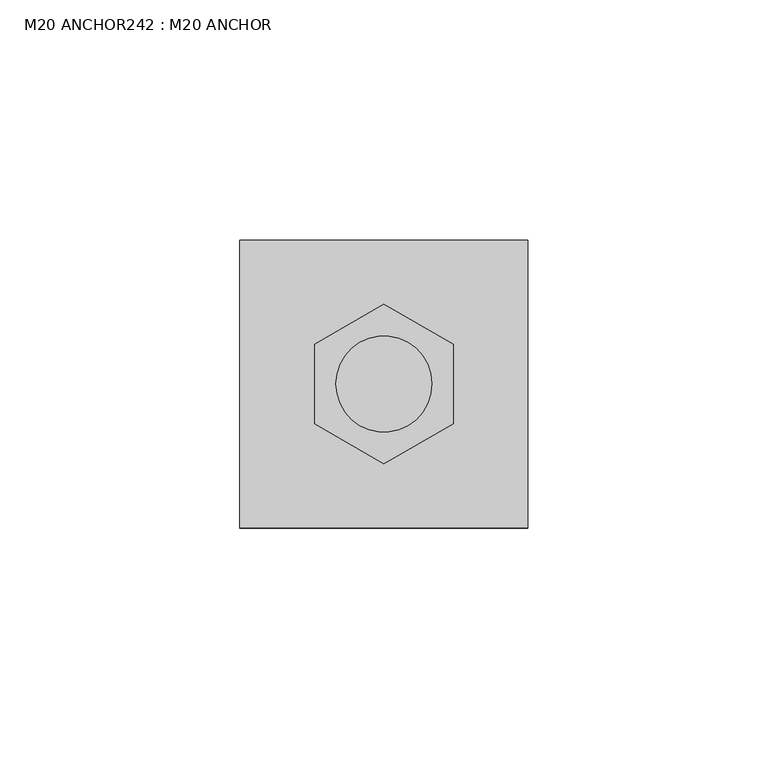
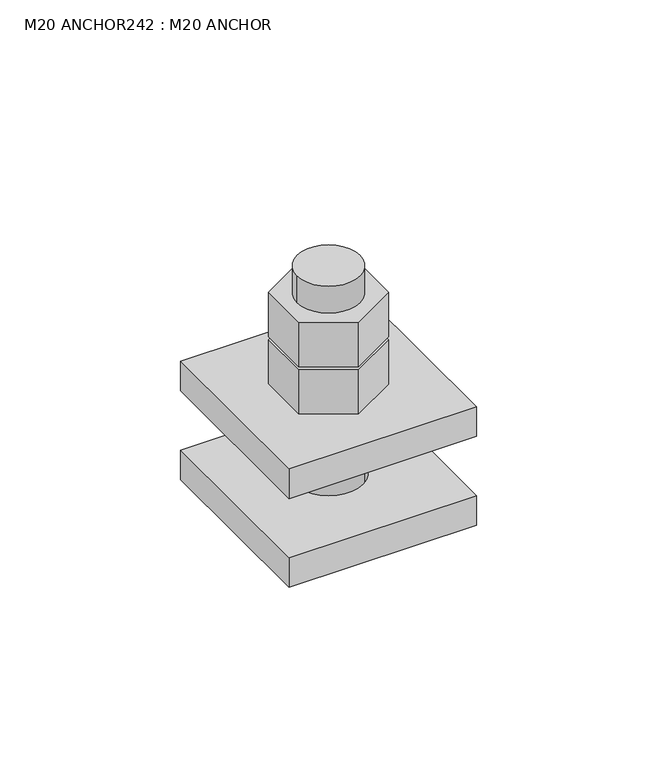
"""IFC4 building model written with IfcOpenShell, lengths in millimetres: fastener geometry, M20 ANCHOR242 : M20 ANCHOR."""

from ifc_helpers import new_model, si_unit, point, frame, frame_2d, origin, place, context, project, spatial, polyline, circle_curve, trimmed, segment, composite_curve, outline, extrude, source, transform, mapped, element, save


def m20_anchor242_m20_anchor_8256c240(model_context):
    return source(origin(), model_context, "Body", "SweptSolid", [
        extrude(outline(polyline([(9008.0855968, 22453.9464399), (9008.0855968, 22470.5835027), (9022.4937158, 22478.9020341), (9036.9018348, 22470.5835027), (9036.9018348, 22453.9464399), (9022.4937158, 22445.6279085), (9008.0855968, 22453.9464399)]), holes=[composite_curve([segment(trimmed(circle_curve(frame_2d((9022.4937158, 22462.2649713)), 10.0), [point((9032.4937158, 22462.2649713))], [point((9012.4937158, 22462.2649713))], True, "CARTESIAN"), True, "CONTINUOUS"), segment(trimmed(circle_curve(frame_2d((9022.4937158, 22462.2649713)), 10.0), [point((9012.4937158, 22462.2649713))], [point((9032.4937158, 22462.2649713))], True, "CARTESIAN"), True, "CONTINUOUS")], self_intersect=False)]), frame((0.0, 0.0, 246.0), z_axis=(0.0, 0.0, 1.0), x_axis=(1.0, 0.0, 0.0)), (0.0, 0.0, 1.0), 15.0),
        extrude(outline(polyline([(9008.0855968, 22453.9464399), (9008.0855968, 22470.5835027), (9022.4937158, 22478.9020341), (9036.9018348, 22470.5835027), (9036.9018348, 22453.9464399), (9022.4937158, 22445.6279085), (9008.0855968, 22453.9464399)]), holes=[composite_curve([segment(trimmed(circle_curve(frame_2d((9022.4937158, 22462.2649713)), 10.0), [point((9032.4937158, 22462.2649713))], [point((9012.4937158, 22462.2649713))], True, "CARTESIAN"), True, "CONTINUOUS"), segment(trimmed(circle_curve(frame_2d((9022.4937158, 22462.2649713)), 10.0), [point((9012.4937158, 22462.2649713))], [point((9032.4937158, 22462.2649713))], True, "CARTESIAN"), True, "CONTINUOUS")], self_intersect=False)]), frame((0.0, 0.0, 230.0), z_axis=(0.0, 0.0, 1.0), x_axis=(1.0, 0.0, 0.0)), (0.0, 0.0, 1.0), 15.0),
        extrude(outline(composite_curve([segment(trimmed(circle_curve(frame_2d((9022.4937158, 22462.2649713)), 10.0), [point((9032.4937158, 22462.2649713))], [point((9012.4937158, 22462.2649713))], False, "CARTESIAN"), True, "CONTINUOUS"), segment(trimmed(circle_curve(frame_2d((9022.4937158, 22462.2649713)), 10.0), [point((9012.4937158, 22462.2649713))], [point((9032.4937158, 22462.2649713))], False, "CARTESIAN"), True, "CONTINUOUS")], self_intersect=False)), frame((0.0, 0.0, 190.0), z_axis=(0.0, 0.0, 1.0), x_axis=(1.0, 0.0, 0.0)), (0.0, 0.0, 1.0), 80.0),
        extrude(outline(polyline([(8992.4937158, 22432.2649713), (8992.4937158, 22492.2649713), (9052.4937158, 22492.2649713), (9052.4937158, 22432.2649713), (8992.4937158, 22432.2649713)]), holes=[composite_curve([segment(trimmed(circle_curve(frame_2d((9022.4937158, 22462.2649713)), 11.0), [point((9033.4937158, 22462.2649713))], [point((9011.4937158, 22462.2649713))], True, "CARTESIAN"), True, "CONTINUOUS"), segment(trimmed(circle_curve(frame_2d((9022.4937158, 22462.2649713)), 11.0), [point((9011.4937158, 22462.2649713))], [point((9033.4937158, 22462.2649713))], True, "CARTESIAN"), True, "CONTINUOUS")], self_intersect=False)]), frame((0.0, 0.0, 190.0), z_axis=(0.0, 0.0, 1.0), x_axis=(1.0, 0.0, 0.0)), (0.0, 0.0, 1.0), 10.0),
        extrude(outline(polyline([(8992.4937158, 22432.2649713), (8992.4937158, 22492.2649713), (9052.4937158, 22492.2649713), (9052.4937158, 22432.2649713), (8992.4937158, 22432.2649713)]), holes=[composite_curve([segment(trimmed(circle_curve(frame_2d((9022.4937158, 22462.2649713)), 11.0), [point((9033.4937158, 22462.2649713))], [point((9011.4937158, 22462.2649713))], True, "CARTESIAN"), True, "CONTINUOUS"), segment(trimmed(circle_curve(frame_2d((9022.4937158, 22462.2649713)), 11.0), [point((9011.4937158, 22462.2649713))], [point((9033.4937158, 22462.2649713))], True, "CARTESIAN"), True, "CONTINUOUS")], self_intersect=False)]), frame((0.0, 0.0, 220.0), z_axis=(0.0, 0.0, 1.0), x_axis=(1.0, 0.0, 0.0)), (0.0, 0.0, 1.0), 10.0),
    ])


if __name__ == "__main__":
    model = new_model("IFC4")
    model_context = context("Model", 3, world=origin())
    ifc_project = project(units=[si_unit("LENGTHUNIT", "METRE", prefix="MILLI")], contexts=[model_context])
    site = spatial("IfcSite", under=ifc_project)
    building = spatial("IfcBuilding", under=site)
    placement = place(None, origin())
    m20_anchor242_m20_anchor_shape = m20_anchor242_m20_anchor_8256c240(model_context)
    element("IfcFastener", 1, ObjectType="M20 ANCHOR242 : M20 ANCHOR", at=placement, inside=building, context=model_context, shape_type="MappedRepresentation", body=[
        mapped(m20_anchor242_m20_anchor_shape, transform((0.0, 0.0, 0.0), x_axis=(1.0, 0.0, 0.0), y_axis=(0.0, 1.0, 0.0), z_axis=(0.0, 0.0, 1.0))),
    ])
    save(model, "model.ifc")
